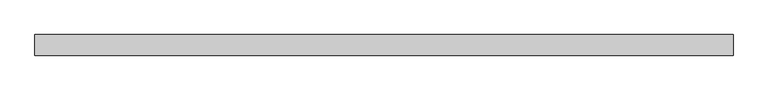
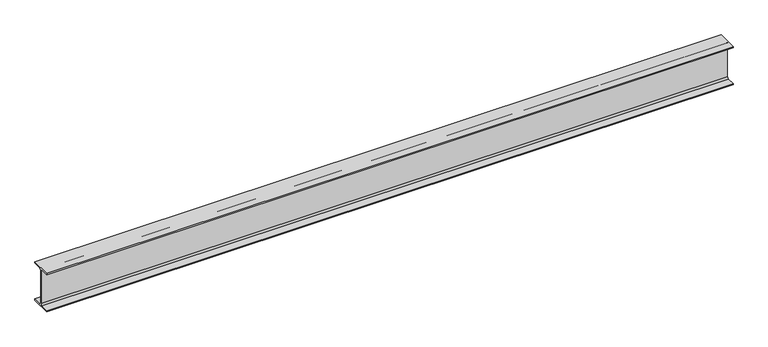
"""IFC4 building model written with IfcOpenShell, lengths in millimetres: beam geometry, 0912_Steel Framing_H-KSD3502 : H_SB_ASB_H-350x175x7x11."""

from ifc_helpers import new_model, si_unit, point, frame, frame_2d, origin, place, context, project, spatial, polyline, circle_curve, trimmed, segment, composite_curve, outline, extrude, source, transform, mapped, element, save


def beam_ba21115e(model_context):
    return source(origin(), model_context, "Body", "SweptSolid", [
        extrude(outline(composite_curve([segment(polyline([(87.5, -164.0), (87.5, -175.0), (-87.5, -175.0), (-87.5, -164.0), (-17.5, -164.0)]), True, "CONTINUOUS"), segment(trimmed(circle_curve(frame_2d((-17.5, -150.0)), 14.0), [point((-17.5, -164.0))], [point((-3.5, -150.0))], True, "CARTESIAN"), True, "CONTINUOUS"), segment(polyline([(-3.5, -150.0), (-3.5, 150.0)]), True, "CONTINUOUS"), segment(trimmed(circle_curve(frame_2d((-17.5, 150.0)), 14.0), [point((-3.5, 150.0))], [point((-17.5, 164.0))], True, "CARTESIAN"), True, "CONTINUOUS"), segment(polyline([(-17.5, 164.0), (-87.5, 164.0), (-87.5, 175.0), (87.5, 175.0), (87.5, 164.0), (17.5, 164.0)]), True, "CONTINUOUS"), segment(trimmed(circle_curve(frame_2d((17.5, 150.0)), 14.0), [point((17.5, 164.0))], [point((3.5, 150.0))], True, "CARTESIAN"), True, "CONTINUOUS"), segment(polyline([(3.5, 150.0), (3.5, -150.0)]), True, "CONTINUOUS"), segment(trimmed(circle_curve(frame_2d((17.5, -150.0)), 14.0), [point((3.5, -150.0))], [point((17.5, -164.0))], True, "CARTESIAN"), True, "CONTINUOUS"), segment(polyline([(17.5, -164.0), (87.5, -164.0)]), True, "CONTINUOUS")], self_intersect=False)), frame((-2898.0326644, 0.0, 0.0), z_axis=(1.0, 0.0, 0.0), x_axis=(0.0, 1.0, 0.0)), (0.0, 0.0, 1.0), 5920.9678677),
    ])


if __name__ == "__main__":
    model = new_model("IFC4")
    model_context = context("Model", 3, world=origin())
    ifc_project = project(units=[si_unit("LENGTHUNIT", "METRE", prefix="MILLI")], contexts=[model_context])
    site = spatial("IfcSite", under=ifc_project)
    building = spatial("IfcBuilding", under=site)
    placement = place(None, origin())
    beam_shape = beam_ba21115e(model_context)
    element("IfcBeam", 1, ObjectType="0912_Steel Framing_H-KSD3502 : H_SB_ASB_H-350x175x7x11", at=placement, inside=building, context=model_context, shape_type="MappedRepresentation", body=[
        mapped(beam_shape, transform((0.0, 0.0, 0.0), x_axis=(1.0, 0.0, 0.0), y_axis=(0.0, 1.0, 0.0), z_axis=(0.0, 0.0, 1.0))),
    ])
    save(model, "model.ifc")

# Revit data of these elements
# Type "0912_Steel Framing_H-KSD3502 : H_SB_ASB_H-350x175x7x11"
#   H_WM Code_1 = "S01AA002-00001 | Main Steel Structure Fabrication Work | Shelter/Building | Medium Steel - Standard (90KG/M>Weight≥30KG/M) | Material: (   )"
#   H_WM Code_2 = "S03AA028-00001 | Main Steel Structure Erection Work | Shelter/Building | Medium Steel (90KG/M>Weight≥30KG/M) | Material: (   )"
#   H_WM Code_3 = "S01AA010-00001 | Main Steel Structure Fabrication Work | Shelter/Building | Steel Painting/Coating | for Non-Fireproofed Steel Surface, Surface Preparation, Primer, Second & Final Coat | Material: (   )"
#   H_Q'ty Cal Type Tag = "SB-Q2"
#   Width = 17.5 cm
#   Web Thickness = 0.7 cm
#   Web Fillet = 1.4 cm
#   Warping Constant = 282000.0 cm⁶
#   W = 0
#   Torsional Moment of Inertia = 19.4042 cm⁴
#   Section Area = 63.14 cm²
#   Plastic Modulus weak axis = 174.0 cm³
#   Plastic Modulus strong axis = 868.0 cm³
#   Perimeter = 1.36 m²/m
#   Nominal Weight = 49.60 kgf/m
#   Moment of Inertia weak axis = 984.00 cm⁴
#   Moment of Inertia strong axis = 13600.00 cm⁴
#   Height = 35.0 cm
#   Flange Thickness = 1.1 cm
#   Elastic Modulus weak axis = 112.0 cm³
#   Elastic Modulus strong axis = 775.0 cm³
#   Centroid Vertical = 17.5 cm
#   Centroid Horizontal = 8.75 cm
#   Ix = 136000000
#   Length [instance default] = 1.5240 m
#   Zx = 868000
#   b = 0.1750 m
#   h = 0.3500 m
#   r = 0.0140 m
#   s = 0.0070 m
#   t = 0.0110 m
#   A = 0.006314 m²
#   Structural Material [instance default] = Steel, 45-345
#   Assembly Code = ""
# Element 1 (IfcBeam, "0912_Steel Framing_H-KSD3502 : H_SB_ASB_H-350x175x7x11")
#   Structural Material = none
# Materials
#   "Steel, 45-345": class "Metal", colour RGB 189 187 185, transparency 0, Description = "Steel 345 MPa", Cost = 0
